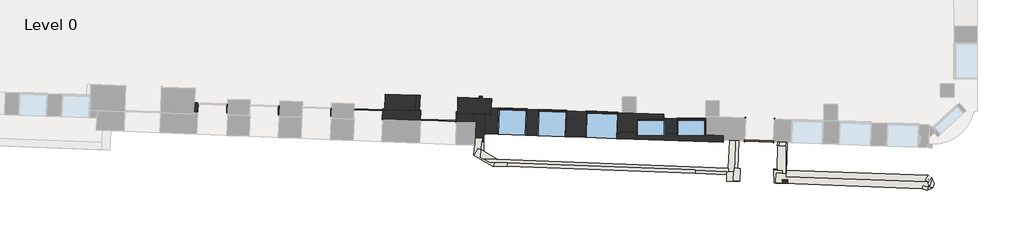
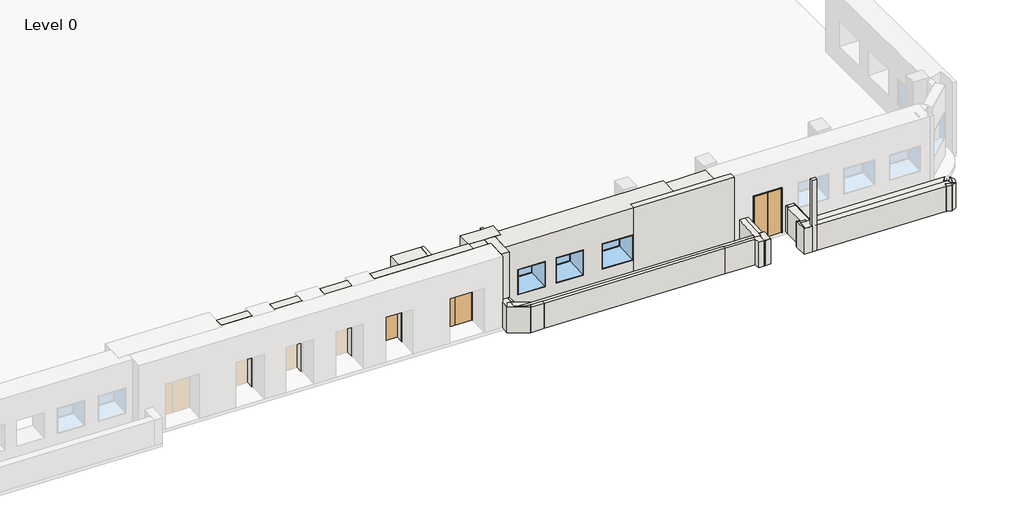
# One storey, part 2 of 9: 37 walls, 5 windows, 3 doors.
# Revit data of these elements (continued)
# Project information
#   Building Name = "Building Name"
#   Workset = "Project Info"
#   Project Issue Date = "06/29/2018"
#   WW-ProjectAddress = "55 Colmore Row"
#   WW-ProjectMarketName = "Birmingham"
#   WW-TemplateVersion = "1.8.48"
# Grids (mm)
#   "1": line (8.8, -29135.916) -> (8.8, 52795.172)
#   "2": line (7418, -29135.916) -> (7418, 52795.172)
#   "3": line (14824.8, -29135.916) -> (14824.8, 52795.172)
#   "4": line (22368, -29135.916) -> (22368, 52795.172)
#   "5": line (34668, -29135.916) -> (34668, 52795.172)
#   "6": line (42195.508, -29135.916) -> (42195.508, 52795.172)
#   "7": line (48145.508, -29135.916) -> (48145.508, 52795.172)
#   "8": line (53958.8, -29135.916) -> (53958.8, 52795.172)
#   "F": line (-24725.375, 205) -> (87660.713, 205)
#   "D": line (-24725.375, 15203.432) -> (87660.713, 15203.432)
#   "E": line (-24725.375, 7713.8) -> (87660.713, 7713.8)
#   "A": line (-24725.375, 38129.775) -> (87660.713, 38129.775)
#   "B": line (-24725.375, 30205) -> (87660.713, 30205)
#   "C": line (-24725.375, 21213.8) -> (87660.713, 21213.8)
# Type "WWm-SingleSolid-Flush : 1200x2100mm"
#   Type Mark = "EX1-55"
#   Construction Type Id = "MDOOR"
#   Assembly Code = "C1020"
#   Analytic Construction = "Metal"
#   Thickness = 50 mm
#   Thermal Resistance (R) = 0.270117 (m²·K)/W
#   Heat Transfer Coefficient (U) = 3.7021 W/(m²·K)
#   Height = 2100 mm
#   Trim Projection Ext = 30 mm
#   Trim Projection Int = 30 mm
#   Trim Width = 25 mm
#   Width = 1200 mm
#   Not 90 Degree [instance default] = no
#   90 Degree [instance default] = yes
#   Door Material = WW-EC-RGB-White
#   Frame Material = WW-EC-RGB-White
#   Visual Light Transmittance = 0
#   Solar Heat Gain Coefficient = 0
#   Function = (empty or 0)
#   Wall Closure = (empty or 0)
# Type "WWm-DoubleSolid-Flush : 1200x2100mm"
#   Type Mark = "EX1-41"
#   Construction Type Id = "MDOOR"
#   Assembly Code = "C1020"
#   Analytic Construction = "Metal"
#   Thickness = 50 mm
#   Thermal Resistance (R) = 0.270117 (m²·K)/W
#   Heat Transfer Coefficient (U) = 3.7021 W/(m²·K)
#   Height = 2100 mm
#   Trim Projection Ext = 25 mm
#   Trim Projection Int = 25 mm
#   Trim Width = 25 mm
#   Width = 1200 mm
#   Not 90 Degree [instance default] = no
#   90 Degree [instance default] = yes
#   Door Material = WW-EC-RGB-White
#   Frame Material = WW-EC-RGB-White
#   Visual Light Transmittance = 0
#   Solar Heat Gain Coefficient = 0
#   Function = (empty or 0)
#   Wall Closure = (empty or 0)
# Type "WWm-DoubleSolid-Flush : 1500x2100mm"
#   Type Mark = "EX1-56"
#   Construction Type Id = "MDOOR"
#   Assembly Code = "C1020"
#   Analytic Construction = "Metal"
#   Thickness = 50 mm
#   Thermal Resistance (R) = 0.270117 (m²·K)/W
#   Heat Transfer Coefficient (U) = 3.7021 W/(m²·K)
#   Height = 2100 mm
#   Trim Projection Ext = 25 mm
#   Trim Projection Int = 25 mm
#   Trim Width = 25 mm
#   Width = 1500 mm
#   Not 90 Degree [instance default] = no
#   90 Degree [instance default] = yes
#   Door Material = WW-EC-RGB-White
#   Frame Material = WW-EC-RGB-White
#   Visual Light Transmittance = 0
#   Solar Heat Gain Coefficient = 0
#   Function = (empty or 0)
#   Wall Closure = (empty or 0)
# Type "WWm-Existing-ExtPartition-715mm"
#   Keynote = ""
#   Type IfcGUID = ""
#   Type Comments = ""
#   Description = ""
#   Type Mark = ""
#   Fire Rating = ""
#   Layers, outside or top first: 715 mm "WW-EC-RGB-White" (function 1)
# Type "WWm-Existing-ExtPartition-1085mm"
#   Keynote = ""
#   Type IfcGUID = ""
#   Type Comments = ""
#   Description = ""
#   Type Mark = ""
#   Fire Rating = ""
#   Layers, outside or top first: 1085 mm "WW-EC-RGB-White" (function 1)
# Type "WWm-Existing-ExtPartition-660mm"
#   Keynote = ""
#   Type IfcGUID = ""
#   Type Comments = ""
#   Description = ""
#   Type Mark = ""
#   Fire Rating = ""
#   Layers, outside or top first: 660 mm "WW-EC-RGB-White" (function 1)
# Type "WWm-Existing-ExtPartition-150mm"
#   Keynote = ""
#   Type IfcGUID = ""
#   Type Comments = ""
#   Description = ""
#   Type Mark = ""
#   Fire Rating = ""
#   Layers, outside or top first: 150 mm "WW-EC-RGB-White" (function 1)
# Type "WWm-Existing-ExtPartition-420mm"
#   Keynote = ""
#   Type IfcGUID = ""
#   Type Comments = ""
#   Description = ""
#   Type Mark = ""
#   Fire Rating = ""
#   Layers, outside or top first: 420 mm "WW-EC-RGB-White" (function 1)
# Type "WWm-Existing-ExtPartition-350mm"
#   Keynote = ""
#   Type IfcGUID = ""
#   Type Comments = ""
#   Description = ""
#   Type Mark = ""
#   Fire Rating = ""
#   Layers, outside or top first: 350 mm "WW-EC-RGB-White" (function 1)
# Type "WWm-Existing-ExtPartition-290mm"
#   Keynote = ""
#   Type IfcGUID = ""
#   Type Comments = ""
#   Description = ""
#   Type Mark = ""
#   Fire Rating = ""
#   Layers, outside or top first: 290 mm "WW-EC-RGB-White" (function 1)
# Type "WWm-Existing-ExtPartition-250mm"
#   Keynote = ""
#   Type IfcGUID = ""
#   Type Comments = ""
#   Description = ""
#   Type Mark = ""
#   Fire Rating = ""
#   Layers, outside or top first: 250 mm "WW-EC-RGB-White" (function 1)
# Type "WWm-Existing-ExtPartition-705mm"
#   Keynote = ""
#   Type IfcGUID = ""
#   Type Comments = ""
#   Description = ""
#   Type Mark = ""
#   Fire Rating = ""
#   Layers, outside or top first: 705 mm "WW-EC-RGB-White" (function 1)
# Type "WWm-Existing-ExtPartition-125mm"
#   Keynote = ""
#   Type IfcGUID = ""
#   Type Comments = ""
#   Description = ""
#   Type Mark = ""
#   Fire Rating = ""
#   Layers, outside or top first: 125 mm "WW-EC-RGB-White" (function 1)
# Type "WWm-Existing-ExtPartition-45mm"
#   Keynote = ""
#   Type IfcGUID = ""
#   Type Comments = ""
#   Description = ""
#   Type Mark = ""
#   Fire Rating = ""
#   Layers, outside or top first: 45 mm "WW-EC-RGB-White" (function 1)
# Type "WWm-Existing-ExtPartition-60mm"
#   Keynote = ""
#   Type IfcGUID = ""
#   Type Comments = ""
#   Description = ""
#   Type Mark = ""
#   Fire Rating = ""
#   Layers, outside or top first: 60 mm "WW-EC-RGB-White" (function 1)
# Type "WWm-Existing-ExtPartition-120mm"
#   Keynote = ""
#   Type IfcGUID = ""
#   Type Comments = ""
#   Description = ""
#   Type Mark = ""
#   Fire Rating = ""
#   Layers, outside or top first: 120 mm "WW-EC-RGB-White" (function 1)
# Type "WWm-Existing-ExtPartition-390mm"
#   Keynote = ""
#   Type IfcGUID = ""
#   Type Comments = ""
#   Description = ""
#   Type Mark = ""
#   Fire Rating = ""
#   Layers, outside or top first: 390 mm "WW-EC-RGB-White" (function 1)
# Type "Window-Instance : 600x1200"
#   Type Mark = "7"
#   Construction Type Id = "GSP4R"
#   Assembly Code = "B2020100"
#   Analytic Construction = "1/8 in Pilkington single glazing"
#   Visual Light Transmittance = 0.9
#   Thermal Resistance (R) = 0.149095 (m²·K)/W
#   Solar Heat Gain Coefficient = 0.86
#   Heat Transfer Coefficient (U) = 6.70716 W/(m²·K)
#   Height [instance default] = 1200 mm
#   Default Sill Height = 900 mm
#   Width [instance default] = 600 mm
#   Window Inset = 20 mm
#   Glass Pane Material = WW-EC-GL-Storefront
#   Sash Material = WW-EC-RGB-White
#   Wall Closure = (empty or 0)
# Element 1 (IfcDoor, "WWm-SingleSolid-Flush : 1200x2100mm")
#   Not 90 Degree = no
#   90 Degree = yes
#   Phase Created = Existing
#   Materials on its faces: "WW-EC-RGB-White"
# Element 2 (IfcDoor, "WWm-DoubleSolid-Flush : 1200x2100mm")
#   Not 90 Degree = no
#   90 Degree = yes
#   Phase Created = Existing
#   Materials on its faces: "WW-EC-RGB-White"
# Element 3 (IfcDoor, "WWm-DoubleSolid-Flush : 1500x2100mm")
#   Not 90 Degree = no
#   90 Degree = yes
#   Phase Created = Existing
#   Materials on its faces: "WW-EC-RGB-White"
# Element 4 (IfcWall, "WWm-Existing-ExtPartition-715mm")
#   Top Offset = -150 mm
#   Base Offset = 0 mm
#   wall height = 3350 mm
#   Phase Created = Existing
#   Base Constraint = Level 0
#   Top Constraint = Level 1
#   Materials on its faces: "WW-EC-RGB-White"
# Elements 5, 9 (IfcWall, "WWm-Existing-ExtPartition-1085mm")
#   Top Offset = -150 mm
#   Base Offset = 0 mm
#   wall height = 3350 mm
#   Phase Created = Existing
#   Base Constraint = Level 0
#   Top Constraint = Level 1
#   Materials on its faces: "WW-EC-RGB-White"
# Elements 6, 7 (IfcWall, "WWm-Existing-ExtPartition-660mm")
#   Top Offset = -150 mm
#   Base Offset = 0 mm
#   wall height = 3350 mm
#   Phase Created = Existing
#   Base Constraint = Level 0
#   Top Constraint = Level 1
#   Materials on its faces: "WW-EC-RGB-White"
# Elements 8, 12 (IfcWall, "WWm-Existing-ExtPartition-150mm")
#   Top Offset = -150 mm
#   Base Offset = 0 mm
#   wall height = 3350 mm
#   Phase Created = Existing
#   Base Constraint = Level 0
#   Top Constraint = Level 1
#   Materials on its faces: "WW-EC-RGB-White"
# Element 10 (IfcWall, "WWm-Existing-ExtPartition-420mm")
#   Top Offset = 0 mm
#   Base Offset = 0 mm
#   Unconnected Height = 1200 mm
#   wall height = 1200 mm
#   Phase Created = Existing
#   Base Constraint = Level 0
#   Materials on its faces: "WW-EC-RGB-White"
# Elements 11, 33, 35 (IfcWall, "WWm-Existing-ExtPartition-350mm")
#   Top Offset = 0 mm
#   Base Offset = 0 mm
#   Unconnected Height = 1200 mm
#   wall height = 1200 mm
#   Phase Created = Existing
#   Base Constraint = Level 0
#   Materials on its faces: "WW-EC-RGB-White"
# Elements 13, 14, 17, 27, 28, 29, 36, 37, 38 (IfcWall, "WWm-Existing-ExtPartition-150mm")
#   Top Offset = 0 mm
#   Base Offset = 0 mm
#   Unconnected Height = 1200 mm
#   wall height = 1200 mm
#   Phase Created = Existing
#   Base Constraint = Level 0
#   Materials on its faces: "WW-EC-RGB-White"
# Elements 15, 18, 24, 25, 32 (IfcWall, "WWm-Existing-ExtPartition-290mm")
#   Top Offset = 0 mm
#   Base Offset = 0 mm
#   Unconnected Height = 1200 mm
#   wall height = 1200 mm
#   Phase Created = Existing
#   Base Constraint = Level 0
#   Materials on its faces: "WW-EC-RGB-White"
# Elements 16, 19, 31 (IfcWall, "WWm-Existing-ExtPartition-250mm")
#   Top Offset = 0 mm
#   Base Offset = 0 mm
#   Unconnected Height = 1200 mm
#   wall height = 1200 mm
#   Phase Created = Existing
#   Base Constraint = Level 0
#   Materials on its faces: "WW-EC-RGB-White"
# Element 20 (IfcWall, "WWm-Existing-ExtPartition-705mm")
#   Top Offset = -150 mm
#   Base Offset = 0 mm
#   wall height = 3350 mm
#   Phase Created = Existing
#   Base Constraint = Level 0
#   Top Constraint = Level 1
#   Materials on its faces: "WW-EC-RGB-White"
# Element 21 (IfcWall, "WWm-Existing-ExtPartition-125mm")
#   Top Offset = -150 mm
#   Base Offset = 0 mm
#   wall height = 3350 mm
#   Phase Created = Existing
#   Base Constraint = Level 0
#   Top Constraint = Level 1
#   Materials on its faces: "WW-EC-RGB-White"
# Element 22 (IfcWall, "WWm-Existing-ExtPartition-290mm")
#   Top Offset = -150 mm
#   Base Offset = 0 mm
#   wall height = 3350 mm
#   Phase Created = Existing
#   Base Constraint = Level 0
#   Top Constraint = Level 1
#   Materials on its faces: "WW-EC-RGB-White"
# Elements 23, 34, 39 (IfcWall, "WWm-Existing-ExtPartition-45mm")
#   Top Offset = 0 mm
#   Base Offset = 0 mm
#   Unconnected Height = 1200 mm
#   wall height = 1200 mm
#   Phase Created = Existing
#   Base Constraint = Level 0
#   Materials on its faces: "WW-EC-RGB-White"
# Element 26 (IfcWall, "WWm-Existing-ExtPartition-60mm")
#   Top Offset = 0 mm
#   Base Offset = 0 mm
#   Unconnected Height = 1200 mm
#   wall height = 1200 mm
#   Phase Created = Existing
#   Base Constraint = Level 0
#   Materials on its faces: "WW-EC-RGB-White"
# Element 30 (IfcWall, "WWm-Existing-ExtPartition-120mm")
#   Top Offset = 0 mm
#   Base Offset = 0 mm
#   Unconnected Height = 1200 mm
#   wall height = 1200 mm
#   Phase Created = Existing
#   Base Constraint = Level 0
#   Materials on its faces: "WW-EC-RGB-White"
# Element 40 (IfcWall, "WWm-Existing-ExtPartition-390mm")
#   Top Offset = -150 mm
#   Base Offset = 0 mm
#   wall height = 3350 mm
#   Phase Created = Existing
#   Base Constraint = Level 0
#   Top Constraint = Level 1
#   Materials on its faces: "WW-EC-RGB-White"
# Element 41 (IfcWindow, "Window-Instance : 600x1200")
#   Mark = "39"
#   Width = 1350 mm
#   Height = 1200 mm
#   Phase Created = Existing
#   Materials on its faces: "WW-EC-RGB-White", "WW-EC-GL-Storefront"
# Element 42 (IfcWindow, "Window-Instance : 600x1200")
#   Mark = "37"
#   Width = 1200 mm
#   Height = 1200 mm
#   Phase Created = Existing
#   Materials on its faces: "WW-EC-RGB-White", "WW-EC-GL-Storefront"
# Element 43 (IfcWindow, "Window-Instance : 600x1200")
#   Mark = "38"
#   Width = 1200 mm
#   Height = 1200 mm
#   Phase Created = Existing
#   Materials on its faces: "WW-EC-RGB-White", "WW-EC-GL-Storefront"
# Element 44 (IfcWindow, "Window-Instance : 600x1200")
#   Mark = "40"
#   Width = 1200 mm
#   Height = 1200 mm
#   Phase Created = Existing
#   Materials on its faces: "WW-EC-RGB-White", "WW-EC-GL-Storefront"
# Element 45 (IfcWindow, "Window-Instance : 600x1200")
#   Mark = "41"
#   Width = 1200 mm
#   Height = 1200 mm
#   Phase Created = Existing
#   Materials on its faces: "WW-EC-RGB-White", "WW-EC-GL-Storefront"
# Materials
#   "WW-EC-RGB-White": class "Generic", colour RGB 255 255 255, transparency 0, Comments = "If region requests off-white, swith asset color to RGB 231-228-220", Description = "Generic Color", Cost = 0
#   "WW-EC-GL-Storefront": class "Glass", colour RGB 236 240 239, transparency 0.85, Description = "Storefront Glass", Cost = 0
